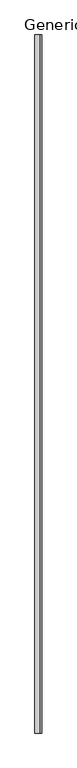
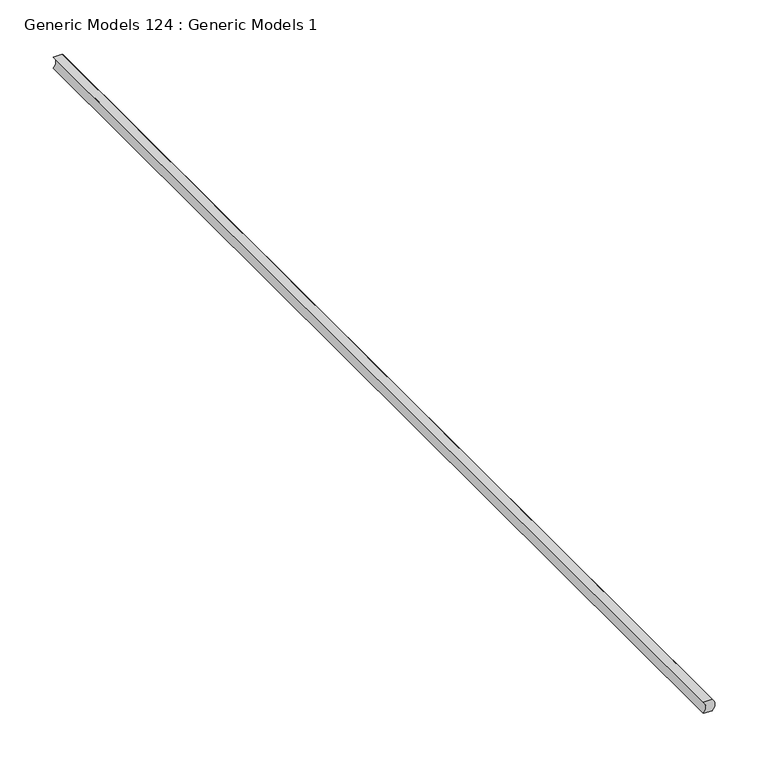
"""IFC4 building model written with IfcOpenShell, lengths in millimetres: proxy geometry, Generic Models 124 : Generic Models 1."""

import ifcopenshell
import ifcopenshell.guid

model = None  # the IFC model being written
_history = None  # IfcOwnerHistory: only IFC2X3 demands one
_inside = {}  # id of a spatial element -> (the spatial element, [elements in it])
_under = {}  # id of a project, library or spatial element -> (it, [spatial elements below it])
_declared = {}  # id of a project -> (the project, [libraries it declares])
_typed = {}  # id of a type object -> (the type object, [elements of that type])
_made_of = {}  # id of a material, layer set ... -> (it, [elements and type objects made of it])


def new_model(schema):
    """Start an empty IFC model of exactly this schema.

    Asked for "IFC4X3", IfcOpenShell would pick the latest addendum, in which some entities
    have other attributes; the version numbers below select the first issue.
    IFC2X3 requires an IfcOwnerHistory on every rooted entity: one is made here for all.
    """
    global model, _history
    if schema == "IFC4X3":
        model = ifcopenshell.file(schema_version=(4, 3, 0, 0))
    else:
        model = ifcopenshell.file(schema=schema)
    _inside.clear()
    _under.clear()
    _declared.clear()
    _typed.clear()
    _made_of.clear()
    _history = None
    if model.schema == "IFC2X3":
        org = make("IfcOrganization", Name="unknown")
        user = make(
            "IfcPersonAndOrganization",
            ThePerson=make("IfcPerson", FamilyName="unknown"),
            TheOrganization=org,
        )
        app = make(
            "IfcApplication",
            ApplicationDeveloper=org,
            Version="unknown",
            ApplicationFullName="unknown",
            ApplicationIdentifier="unknown",
        )
        _history = make(
            "IfcOwnerHistory",
            OwningUser=user,
            OwningApplication=app,
            ChangeAction="ADDED",
            CreationDate=0,
        )
    return model


def make(cls, **values):
    """One entity of the class cls with the attributes given. An attribute that is None is left unset."""
    return model.create_entity(
        cls, **{name: value for name, value in values.items() if value is not None}
    )


def rooted(cls, **values):
    """An entity with a GlobalId (a new one), such as an element, a storey or a relation."""
    return make(cls, GlobalId=ifcopenshell.guid.new(), OwnerHistory=_history, **values)


def si_unit(unit_type, name, prefix=None):
    """IfcSIUnit, for example si_unit("LENGTHUNIT", "METRE", prefix="MILLI")."""
    return make("IfcSIUnit", UnitType=unit_type, Prefix=prefix, Name=name)


def assignment(units):
    """IfcUnitAssignment: the units of a project."""
    return None if units is None else make("IfcUnitAssignment", Units=units)


def point(xyz):
    """IfcCartesianPoint."""
    return None if xyz is None else make("IfcCartesianPoint", Coordinates=xyz)


def direction(xyz):
    """IfcDirection."""
    return None if xyz is None else make("IfcDirection", DirectionRatios=xyz)


def frame(location, z_axis=None, x_axis=None):
    """IfcAxis2Placement3D, a coordinate frame: its origin and axes. An axis left out is left unset."""
    return make(
        "IfcAxis2Placement3D",
        Location=point(location),
        Axis=direction(z_axis),
        RefDirection=direction(x_axis),
    )


def frame_2d(location, x_axis=None):
    """IfcAxis2Placement2D, a coordinate frame in the plane: its origin and x axis."""
    return make(
        "IfcAxis2Placement2D", Location=point(location), RefDirection=direction(x_axis)
    )


def origin():
    """The frame at (0, 0, 0) with its axes left unset."""
    return frame((0.0, 0.0, 0.0))


def place(relative_to, where):
    """IfcLocalPlacement: puts the frame where relative to a parent placement (None: the world)."""
    return make(
        "IfcLocalPlacement", PlacementRelTo=relative_to, RelativePlacement=where
    )


def context(
    kind, dimensions, precision=None, world=None, true_north=None, identifier=None
):
    """IfcGeometricRepresentationContext, for example the 3D "Model" context."""
    return make(
        "IfcGeometricRepresentationContext",
        ContextIdentifier=identifier,
        ContextType=kind,
        CoordinateSpaceDimension=dimensions,
        Precision=precision,
        WorldCoordinateSystem=world,
        TrueNorth=true_north,
    )


def project(units=None, contexts=None):
    """IfcProject with its units and contexts."""
    return rooted(
        "IfcProject",
        Name="project",
        RepresentationContexts=contexts,
        UnitsInContext=assignment(units),
    )


def spatial(cls, under=None, at=None, **own):
    """A site, building, storey or space (cls), placed at a placement, below another one or the project."""
    s = rooted(cls, ObjectPlacement=at, **own)
    if under is not None:
        _under.setdefault(under.id(), (under, []))[1].append(s)
    return s


def polyline(points):
    """IfcPolyline through the points."""
    return make("IfcPolyline", Points=[point(p) for p in points])


def circle_curve(where, radius):
    """IfcCircle in the frame where."""
    return make("IfcCircle", Position=where, Radius=radius)


def trimmed(basis, trim1, trim2, sense, master):
    """IfcTrimmedCurve: the piece of a basis curve between two trims."""
    return make(
        "IfcTrimmedCurve",
        BasisCurve=basis,
        Trim1=trim1,
        Trim2=trim2,
        SenseAgreement=sense,
        MasterRepresentation=master,
    )


def segment(curve, same_sense, transition):
    """IfcCompositeCurveSegment."""
    return make(
        "IfcCompositeCurveSegment",
        Transition=transition,
        SameSense=same_sense,
        ParentCurve=curve,
    )


def composite_curve(segments, self_intersect=None):
    """IfcCompositeCurve: segments joined end to end."""
    return make("IfcCompositeCurve", Segments=segments, SelfIntersect=self_intersect)


def outline(outer, holes=None, kind="AREA"):
    """IfcArbitraryClosedProfileDef: a profile drawn as a closed curve; with holes, ...WithVoids."""
    if holes is None:
        return make("IfcArbitraryClosedProfileDef", ProfileType=kind, OuterCurve=outer)
    return make(
        "IfcArbitraryProfileDefWithVoids",
        ProfileType=kind,
        OuterCurve=outer,
        InnerCurves=holes,
    )


def extrude(swept, where, along, depth):
    """IfcExtrudedAreaSolid: the profile swept, set in the frame where, extruded along a direction by depth."""
    return make(
        "IfcExtrudedAreaSolid",
        SweptArea=swept,
        Position=where,
        ExtrudedDirection=direction(along),
        Depth=depth,
    )


def shape(context_of_items, identifier, shape_type, items):
    """IfcShapeRepresentation: the items that make up one representation, for example the "Body"."""
    return make(
        "IfcShapeRepresentation",
        ContextOfItems=context_of_items,
        RepresentationIdentifier=identifier,
        RepresentationType=shape_type,
        Items=items,
    )


def source(mapping_origin, context_of_items, identifier, shape_type, items):
    """IfcRepresentationMap: a shape defined once, which mapped items show again and again."""
    return make(
        "IfcRepresentationMap",
        MappingOrigin=mapping_origin,
        MappedRepresentation=shape(context_of_items, identifier, shape_type, items),
    )


def transform(
    local_origin,
    x_axis=None,
    y_axis=None,
    z_axis=None,
    scale=None,
    scale2=None,
    scale3=None,
    uniform=True,
):
    """IfcCartesianTransformationOperator3D, or its non-uniform kind. x_axis, y_axis, z_axis: its Axis1, 2, 3."""
    if uniform:
        return make(
            "IfcCartesianTransformationOperator3D",
            Axis1=direction(x_axis),
            Axis2=direction(y_axis),
            LocalOrigin=point(local_origin),
            Scale=scale,
            Axis3=direction(z_axis),
        )
    return make(
        "IfcCartesianTransformationOperator3DnonUniform",
        Axis1=direction(x_axis),
        Axis2=direction(y_axis),
        LocalOrigin=point(local_origin),
        Scale=scale,
        Axis3=direction(z_axis),
        Scale2=scale2,
        Scale3=scale3,
    )


def mapped(mapping_source, mapping_target):
    """IfcMappedItem: shows the shape of a source again, moved by a transform."""
    return make(
        "IfcMappedItem", MappingSource=mapping_source, MappingTarget=mapping_target
    )


def made_of(thing, what):
    """Note that an element or type object is made of a material, layer set ...; save() writes the relation."""
    if what is not None:
        _made_of.setdefault(what.id(), (what, []))[1].append(thing)
    return thing


def element(
    cls,
    number,
    at=None,
    inside=None,
    cuts=None,
    type_object=None,
    material=None,
    context=None,
    identifier="Body",
    shape_type=None,
    held_by="IfcProductDefinitionShape",
    body=None,
    shapes=None,
    **own,
):
    """One element of the class cls, such as IfcWall. Its Tag is "e" and its number.

    at: its placement. inside: the storey or other place that contains it. cuts: it is an
    opening in that element (IfcRelVoidsElement). A single representation is given by context,
    identifier, shape_type and body (its items); several are given by shapes. held_by: the class
    of the entity that holds the representations. save() writes the other relations.
    """
    e = rooted(cls, Tag="e%d" % number, ObjectPlacement=at, **own)
    if body is not None:
        shapes = [shape(context, identifier, shape_type, body)]
    if shapes is not None:
        e.Representation = make(held_by, Representations=shapes)
    if inside is not None:
        _inside.setdefault(inside.id(), (inside, []))[1].append(e)
    if cuts is not None:
        rooted(
            "IfcRelVoidsElement", RelatingBuildingElement=cuts, RelatedOpeningElement=e
        )
    if type_object is not None:
        _typed.setdefault(type_object.id(), (type_object, []))[1].append(e)
    return made_of(e, material)


def aggregate(whole, parts):
    """IfcRelAggregates: a whole, such as a stair, and the parts it consists of."""
    return rooted("IfcRelAggregates", RelatingObject=whole, RelatedObjects=parts)


def save(model, path):
    """Write the relations noted so far, then the file.

    IfcRelAggregates (storeys below a building ...), IfcRelContainedInSpatialStructure (elements
    in a storey), IfcRelDefinesByType, IfcRelAssociatesMaterial and IfcRelDeclares: one each for
    every whole, place, type object, material and project.
    """
    for whole, parts in _under.values():
        aggregate(whole, parts)
    for where, things in _inside.values():
        rooted(
            "IfcRelContainedInSpatialStructure",
            RelatedElements=things,
            RelatingStructure=where,
        )
    for kind, things in _typed.values():
        rooted("IfcRelDefinesByType", RelatedObjects=things, RelatingType=kind)
    for what, things in _made_of.values():
        rooted("IfcRelAssociatesMaterial", RelatedObjects=things, RelatingMaterial=what)
    for by, libraries in _declared.values():
        rooted("IfcRelDeclares", RelatingContext=by, RelatedDefinitions=libraries)
    model.write(path)


def generic_models_124_generic_models_1_3ec1b419(model_context):
    return source(origin(), model_context, "Body", "SweptSolid", [
        extrude(outline(composite_curve([segment(polyline([(294.3266124, 52113.2990371), (294.3266124, 52122.8240371)]), True, "CONTINUOUS"), segment(trimmed(circle_curve(frame_2d((300.6766124, 52116.9945561)), 8.620055), [point((294.3266124, 52122.8240371))], [point((307.0266124, 52122.8240371))], False, "CARTESIAN"), True, "CONTINUOUS"), segment(polyline([(307.0266124, 52122.8240371), (307.0266124, 52113.2990371)]), True, "CONTINUOUS"), segment(trimmed(circle_curve(frame_2d((300.6766124, 52107.4695561)), 8.620055), [point((307.0266124, 52113.2990371))], [point((294.3266124, 52113.2990371))], True, "CARTESIAN"), True, "CONTINUOUS")], self_intersect=False)), frame((0.0, 0.0, 0.0), z_axis=(0.0, 1.0, 0.0), x_axis=(0.0, 0.0, 1.0)), (0.0, 0.0, 1.0), 1219.2),
    ])


if __name__ == "__main__":
    model = new_model("IFC4")
    model_context = context("Model", 3, world=origin())
    ifc_project = project(units=[si_unit("LENGTHUNIT", "METRE", prefix="MILLI")], contexts=[model_context])
    site = spatial("IfcSite", under=ifc_project)
    building = spatial("IfcBuilding", under=site)
    placement = place(None, origin())
    generic_models_124_generic_models_1_shape = generic_models_124_generic_models_1_3ec1b419(model_context)
    element("IfcBuildingElementProxy", 1, Name="Generic Models 124 : Generic Models 1", ObjectType="Generic Models 124 : Generic Models 1", at=placement, inside=building, context=model_context, shape_type="MappedRepresentation", body=[
        mapped(generic_models_124_generic_models_1_shape, transform((0.0, 0.0, 0.0), x_axis=(1.0, 0.0, 0.0), y_axis=(0.0, 1.0, 0.0), z_axis=(0.0, 0.0, 1.0))),
    ])
    save(model, "model.ifc")

# Revit data of these elements
# Element 1 (IfcBuildingElementProxy, "Generic Models 124 : Generic Models 1")
#   Materials on its faces: "SEALANT (W/ BACKER ROD IF NECESSARY)"
# Materials
#   "SEALANT (W/ BACKER ROD IF NECESSARY)": class "Unassigned", colour RGB 120 120 120, transparency 0, Cost = 0
